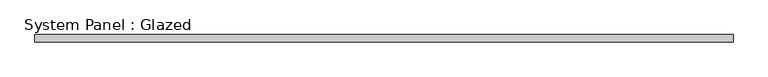
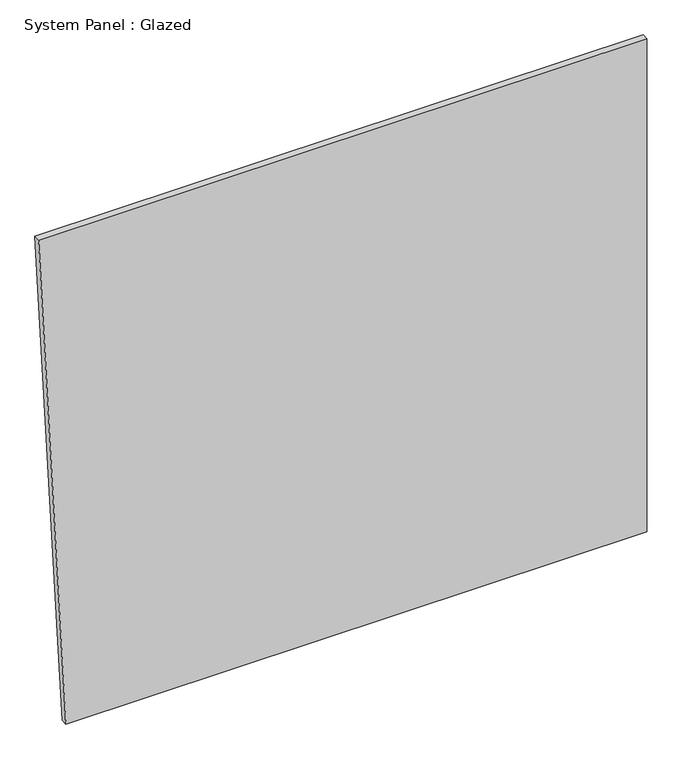
"""IFC4 building model written with IfcOpenShell, lengths in millimetres: plate geometry, System Panel : Glazed."""

from ifc_helpers import new_model, si_unit, frame, origin, place, context, project, spatial, polyline, outline, extrude, source, transform, mapped, element, save


def system_panel_glazed_e065ae4e(model_context):
    return source(origin(), model_context, "Body", "SweptSolid", [
        extrude(outline(polyline([(0.0, -1108.2089886), (0.0, 1217.3908418), (2086.1728929, 1217.3908418), (2086.1728929, -1217.3908418), (0.0, -1108.2089886)])), frame((0.0, -44.45, 0.0), z_axis=(0.0, 1.0, 0.0), x_axis=(0.0, 0.0, 1.0)), (0.0, 0.0, 1.0), 25.4),
    ])


if __name__ == "__main__":
    model = new_model("IFC4")
    model_context = context("Model", 3, world=origin())
    ifc_project = project(units=[si_unit("LENGTHUNIT", "METRE", prefix="MILLI")], contexts=[model_context])
    site = spatial("IfcSite", under=ifc_project)
    building = spatial("IfcBuilding", under=site)
    placement = place(None, origin())
    system_panel_glazed_shape = system_panel_glazed_e065ae4e(model_context)
    element("IfcPlate", 1, ObjectType="System Panel : Glazed", at=placement, inside=building, context=model_context, shape_type="MappedRepresentation", body=[
        mapped(system_panel_glazed_shape, transform((0.0, 0.0, 0.0), x_axis=(1.0, 0.0, 0.0), y_axis=(0.0, 1.0, 0.0), z_axis=(0.0, 0.0, 1.0))),
    ])
    save(model, "model.ifc")

# Revit data of these elements
# Type "System Panel : Glazed"
#   Construction Type Id = "GSP4R"
#   Analytic Construction = "1/8 in Pilkington single glazing"
#   Visual Light Transmittance = 0.9
#   Solar Heat Gain Coefficient = 0.86
#   Heat Transfer Coefficient (U) = 1.18115 BTU/(h·ft²·°F)
#   Define Thermal Properties by = 1
# Element 1 (IfcPlate, "System Panel : Glazed")
#   Materials on its faces: "Glass"
# Materials
#   "Glass": class "Glass", colour RGB 0 128 192, transparency 0.75, Description = "Soda Lime Glass", Cost = 0
